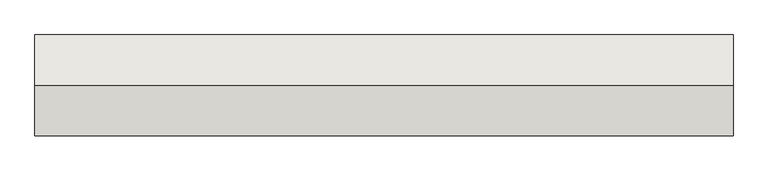
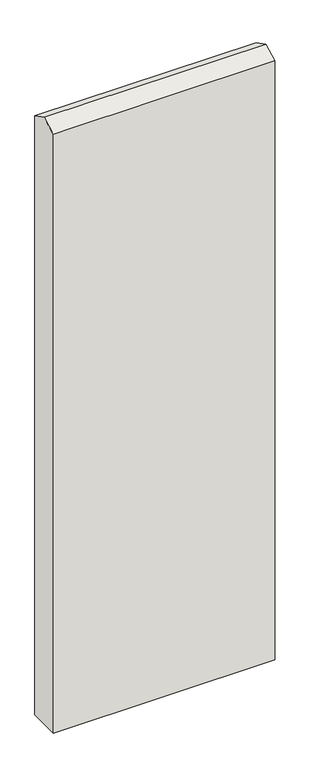
"""IFC4 building model written with IfcOpenShell, lengths in millimetres: wall geometry, Holzwand."""

from ifc_helpers import new_model, si_unit, frame, origin, place, context, project, spatial, polyline, outline, extrude, source, transform, mapped, element, save


def wall_3d8a0fa4(model_context):
    return source(origin(), model_context, "Body", "SweptSolid", [
        extrude(outline(polyline([(100.0, 4011.6781465), (200.0, 3960.7256015), (200.0, 0.0), (0.0, 0.0), (0.0, 3960.7256015), (100.0, 4011.6781465)])), frame((0.0, 0.0, 0.0), z_axis=(1.0, 0.0, 0.0), x_axis=(0.0, 1.0, 0.0)), (0.0, 0.0, 1.0), 1385.0),
    ])


if __name__ == "__main__":
    model = new_model("IFC4")
    model_context = context("Model", 3, world=origin())
    ifc_project = project(units=[si_unit("LENGTHUNIT", "METRE", prefix="MILLI")], contexts=[model_context])
    site = spatial("IfcSite", under=ifc_project)
    building = spatial("IfcBuilding", under=site)
    placement = place(None, origin())
    wall_shape = wall_3d8a0fa4(model_context)
    element("IfcWall", 1, ObjectType="Holzwand", at=placement, inside=building, context=model_context, shape_type="MappedRepresentation", body=[
        mapped(wall_shape, transform((0.0, 0.0, 0.0), x_axis=(1.0, 0.0, 0.0), y_axis=(0.0, 1.0, 0.0), z_axis=(0.0, 0.0, 1.0))),
    ])
    save(model, "model.ifc")

# Revit data of these elements
# Element 1 (IfcWall, "Holzwand")
#   Materials on its faces: "holzschalung"
# Materials
#   "holzschalung": class "Unassigned", colour RGB 128 128 128, transparency 0
